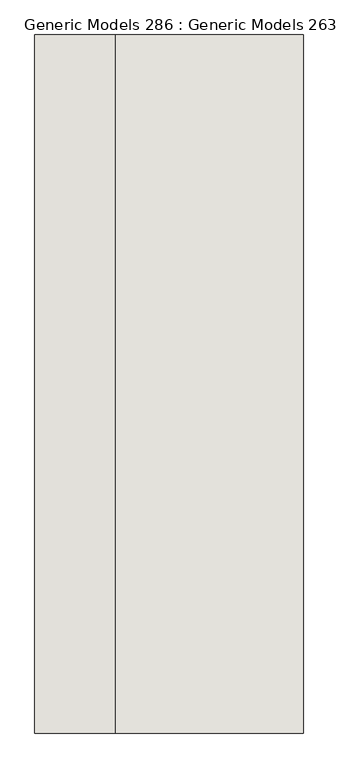
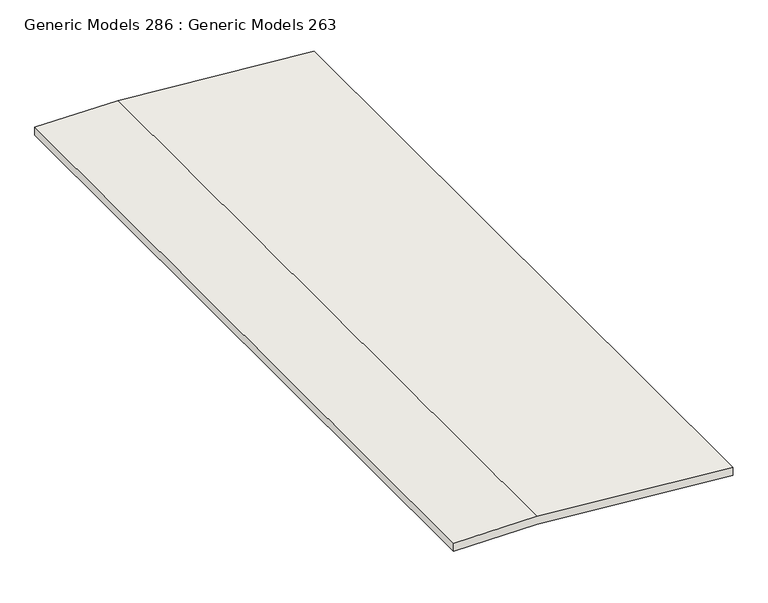
"""IFC4 building model written with IfcOpenShell, lengths in millimetres: wall geometry, Generic Models 286 : Generic Models 263."""

from ifc_helpers import new_model, si_unit, frame, origin, place, context, project, spatial, polyline, outline, extrude, source, transform, mapped, element, save


def generic_models_286_generic_models_263_54c6d84c(model_context):
    return source(origin(), model_context, "Body", "SweptSolid", [
        extrude(outline(polyline([(-18.0020399, 88031.3862389), (0.2818898, 86515.9481279), (-152.129202, 86515.9481279), (-170.3245887, 88024.0474769), (-470.5124436, 91579.9797726), (-317.5703646, 91579.9797726), (-18.0020399, 88031.3862389)])), frame((0.0, -9654.7737439, 0.0), z_axis=(0.0, 1.0, 0.0), x_axis=(0.0, 0.0, 1.0)), (0.0, 0.0, 1.0), 13159.4929723),
    ])


if __name__ == "__main__":
    model = new_model("IFC4")
    model_context = context("Model", 3, world=origin())
    ifc_project = project(units=[si_unit("LENGTHUNIT", "METRE", prefix="MILLI")], contexts=[model_context])
    site = spatial("IfcSite", under=ifc_project)
    building = spatial("IfcBuilding", under=site)
    placement = place(None, origin())
    generic_models_286_generic_models_263_shape = generic_models_286_generic_models_263_54c6d84c(model_context)
    element("IfcWall", 1, ObjectType="Generic Models 286 : Generic Models 263", at=placement, inside=building, context=model_context, shape_type="MappedRepresentation", body=[
        mapped(generic_models_286_generic_models_263_shape, transform((0.0, 0.0, 0.0), x_axis=(1.0, 0.0, 0.0), y_axis=(0.0, 1.0, 0.0), z_axis=(0.0, 0.0, 1.0))),
    ])
    save(model, "model.ifc")

# Revit data of these elements
# Element 1 (IfcWall, "Generic Models 286 : Generic Models 263")
#   Materials on its faces: "6\" CRUSHED AGGREGATE BASE COURSE"
# Materials
#   "6\" CRUSHED AGGREGATE BASE COURSE": class "Miscellaneous", colour RGB 167 168 186, transparency 0, Cost = 0
